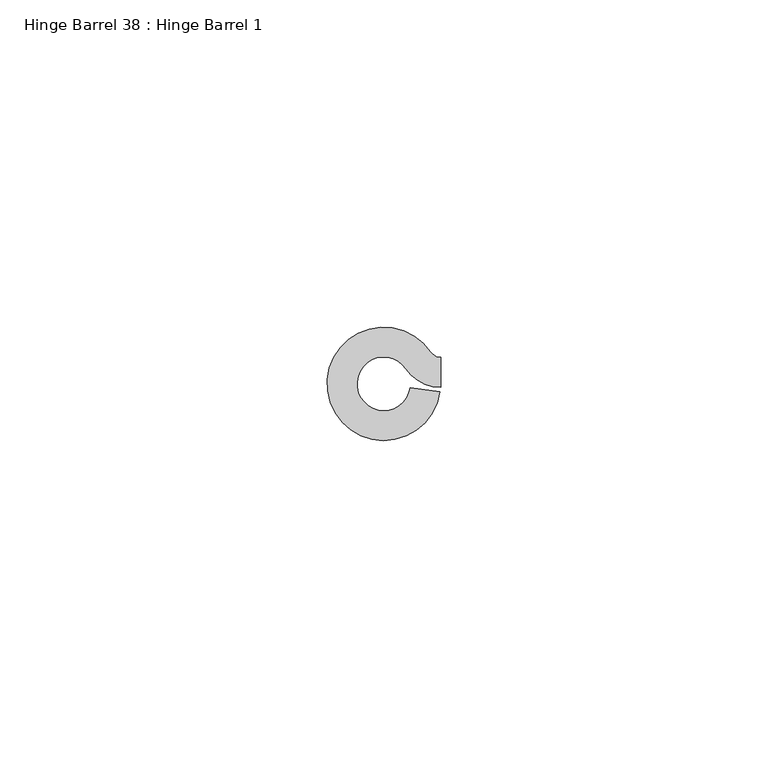
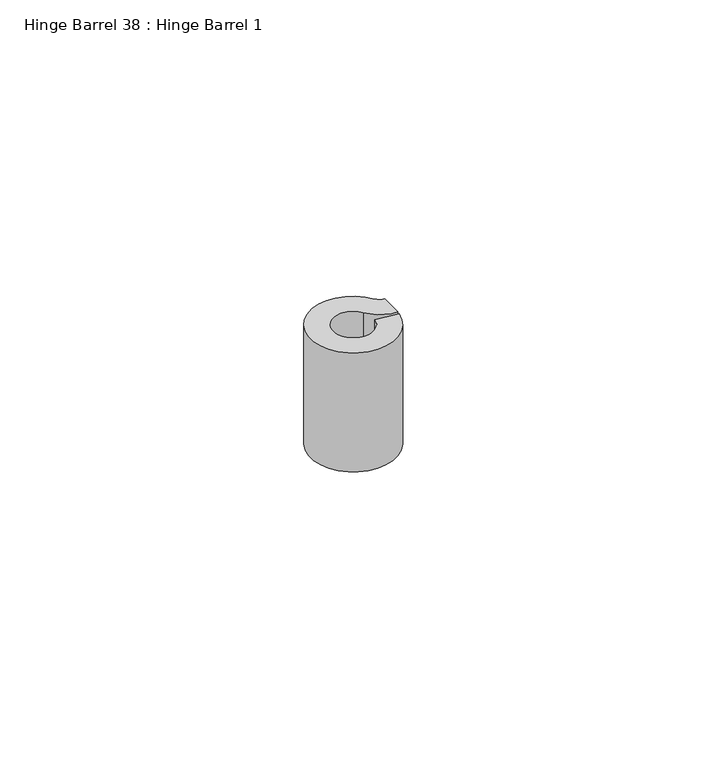
"""IFC4 building model written with IfcOpenShell, lengths in millimetres: proxy geometry, Hinge Barrel 38 : Hinge Barrel 1."""

from ifc_helpers import new_model, si_unit, point, frame, frame_2d, origin, place, context, project, spatial, polyline, circle_curve, trimmed, segment, composite_curve, outline, extrude, source, transform, mapped, element, save


def hinge_barrel_38_hinge_barrel_1_d177c79a(model_context):
    return source(origin(), model_context, "Body", "SweptSolid", [
        extrude(outline(composite_curve([segment(trimmed(circle_curve(frame_2d((587319.1320739, -534100.7049841)), 4.0894), [point((587322.5194669, -534098.4139665))], [point((587323.1821338, -534101.2708529))], True, "CARTESIAN"), True, "CONTINUOUS"), segment(polyline([(587323.1821338, -534101.2708529), (587327.7022899, -534101.9024028)]), True, "CONTINUOUS"), segment(trimmed(circle_curve(frame_2d((587319.1320739, -534100.7049841)), 8.6534625), [point((587327.7022899, -534101.9024028))], [point((587326.3000393, -534095.8570273))], False, "CARTESIAN"), True, "CONTINUOUS"), segment(trimmed(circle_curve(frame_2d((587327.8245257, -534094.8259615)), 1.8404226), [point((587326.3000393, -534095.8570273))], [point((587327.8245257, -534096.6663841))], True, "CARTESIAN"), True, "CONTINUOUS"), segment(polyline([(587327.8245257, -534096.6663841), (587327.8245257, -534101.2304466)]), True, "CONTINUOUS"), segment(trimmed(circle_curve(frame_2d((587327.8245257, -534094.8259615)), 6.4044851), [point((587327.8245257, -534101.2304466))], [point((587322.5194669, -534098.4139665))], False, "CARTESIAN"), True, "CONTINUOUS")], self_intersect=False)), frame((0.0, 0.0, 336.55), z_axis=(0.0, 0.0, 1.0), x_axis=(1.0, 0.0, 0.0)), (0.0, 0.0, 1.0), 25.4),
    ])


if __name__ == "__main__":
    model = new_model("IFC4")
    model_context = context("Model", 3, world=origin())
    ifc_project = project(units=[si_unit("LENGTHUNIT", "METRE", prefix="MILLI")], contexts=[model_context])
    site = spatial("IfcSite", under=ifc_project)
    building = spatial("IfcBuilding", under=site)
    placement = place(None, origin())
    hinge_barrel_38_hinge_barrel_1_shape = hinge_barrel_38_hinge_barrel_1_d177c79a(model_context)
    element("IfcBuildingElementProxy", 1, Name="Hinge Barrel 38 : Hinge Barrel 1", ObjectType="Hinge Barrel 38 : Hinge Barrel 1", at=placement, inside=building, context=model_context, shape_type="MappedRepresentation", body=[
        mapped(hinge_barrel_38_hinge_barrel_1_shape, transform((0.0, 0.0, 0.0), x_axis=(1.0, 0.0, 0.0), y_axis=(0.0, 1.0, 0.0), z_axis=(0.0, 0.0, 1.0))),
    ])
    save(model, "model.ifc")

# Revit data of these elements
# Element 1 (IfcBuildingElementProxy, "Hinge Barrel 38 : Hinge Barrel 1")
#   Materials on its faces: "6\"X6\" WELD-ON STL BUTT HINGE"
# Materials
#   "6\"X6\" WELD-ON STL BUTT HINGE": class "Metal", colour RGB 189 187 185, transparency 0, Description = "Carbon steel", Cost = 0
